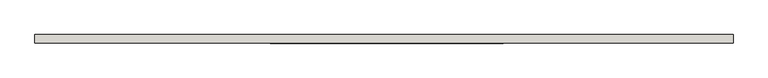
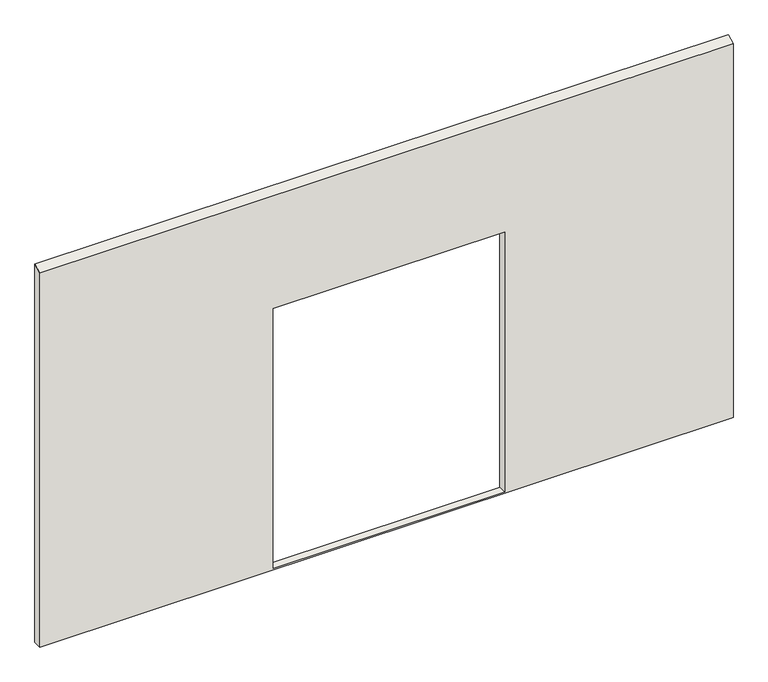
"""IFC4 building model written with IfcOpenShell, lengths in millimetres: wall geometry, 0_3d."""

from ifc_helpers import new_model, si_unit, origin, place, context, project, spatial, faceted_brep, source, transform, mapped, element, save


def wall_c116ed62(model_context):
    return source(origin(), model_context, "Body", "Brep", [
        faceted_brep([(1919.0, 70.0, 10.0), (1919.0, 70.0, 2270.0), (1919.0, 0.0, 2270.0), (1919.0, 0.0, 10.0), (3819.0, 70.0, 2270.0), (3819.0, 0.0, 2270.0), (3819.0, 70.0, 10.0), (3819.0, 0.0, 10.0), (5694.0, 0.0, 3247.913011), (5694.0, 70.0, 3283.5797924), (0.0, 70.0, 3283.5797924), (0.0, 0.0, 3247.913011), (0.0, 70.0, 0.0), (0.0, 0.0, 0.0), (5694.0, 0.0, 0.0), (5694.0, 70.0, 0.0)], [[[0, 1, 2, 3]], [[1, 4, 5, 2]], [[4, 6, 7, 5]], [[6, 0, 3, 7]], [[8, 9, 10, 11]], [[11, 10, 12, 13]], [[9, 8, 14, 15]], [[8, 11, 13, 14], [3, 2, 5, 7]], [[15, 12, 10, 9], [1, 0, 6, 4]], [[12, 15, 14, 13]]]),
    ])


if __name__ == "__main__":
    model = new_model("IFC4")
    model_context = context("Model", 3, world=origin())
    ifc_project = project(units=[si_unit("LENGTHUNIT", "METRE", prefix="MILLI")], contexts=[model_context])
    site = spatial("IfcSite", under=ifc_project)
    building = spatial("IfcBuilding", under=site)
    placement = place(None, origin())
    wall_shape = wall_c116ed62(model_context)
    element("IfcWall", 1, ObjectType="0_3d", at=placement, inside=building, context=model_context, shape_type="MappedRepresentation", body=[
        mapped(wall_shape, transform((0.0, 0.0, 0.0), x_axis=(1.0, 0.0, 0.0), y_axis=(0.0, 1.0, 0.0), z_axis=(0.0, 0.0, 1.0))),
    ])
    save(model, "model.ifc")

# Revit data of these elements
# Element 1 (IfcWall, "0_3d")
#   Materials on its faces: "Glass_Simple"
# Materials
#   "Glass_Simple": class "Unassigned", colour RGB 255 255 255, transparency 0.9
